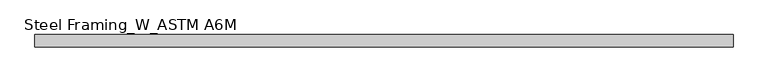
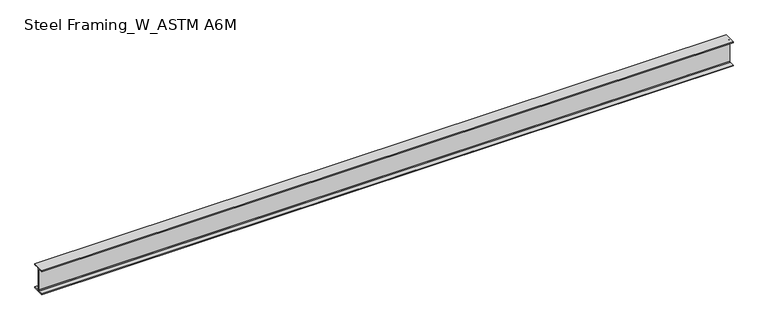
"""IFC4 building model written with IfcOpenShell, lengths in millimetres: beam geometry, Steel Framing_W_ASTM A6M : H_SB_AR_S02_W360x51_B4."""

from ifc_helpers import new_model, si_unit, point, frame, frame_2d, origin, place, context, project, spatial, polyline, circle_curve, trimmed, segment, composite_curve, outline, extrude, source, transform, mapped, element, save


def steel_framing_w_astm_a6m_e8746ce3(model_context):
    return source(origin(), model_context, "Body", "SweptSolid", [
        extrude(outline(composite_curve([segment(polyline([(85.5, -166.4), (85.5, -178.0), (-85.5, -178.0), (-85.5, -166.4), (-13.72, -166.4)]), True, "CONTINUOUS"), segment(trimmed(circle_curve(frame_2d((-13.72, -156.3)), 10.1), [point((-13.72, -166.4))], [point((-3.62, -156.3))], True, "CARTESIAN"), True, "CONTINUOUS"), segment(polyline([(-3.62, -156.3), (-3.62, 156.3)]), True, "CONTINUOUS"), segment(trimmed(circle_curve(frame_2d((-13.72, 156.3)), 10.1), [point((-3.62, 156.3))], [point((-13.72, 166.4))], True, "CARTESIAN"), True, "CONTINUOUS"), segment(polyline([(-13.72, 166.4), (-85.5, 166.4), (-85.5, 178.0), (85.5, 178.0), (85.5, 166.4), (13.72, 166.4)]), True, "CONTINUOUS"), segment(trimmed(circle_curve(frame_2d((13.72, 156.3)), 10.1), [point((13.72, 166.4))], [point((3.62, 156.3))], True, "CARTESIAN"), True, "CONTINUOUS"), segment(polyline([(3.62, 156.3), (3.62, -156.3)]), True, "CONTINUOUS"), segment(trimmed(circle_curve(frame_2d((13.72, -156.3)), 10.1), [point((3.62, -156.3))], [point((13.72, -166.4))], True, "CARTESIAN"), True, "CONTINUOUS"), segment(polyline([(13.72, -166.4), (85.5, -166.4)]), True, "CONTINUOUS")], self_intersect=False)), frame((-4901.8, 0.0, 0.0), z_axis=(1.0, 0.0, 0.0), x_axis=(0.0, 1.0, 0.0)), (0.0, 0.0, 1.0), 9715.9),
    ])


if __name__ == "__main__":
    model = new_model("IFC4")
    model_context = context("Model", 3, world=origin())
    ifc_project = project(units=[si_unit("LENGTHUNIT", "METRE", prefix="MILLI")], contexts=[model_context])
    site = spatial("IfcSite", under=ifc_project)
    building = spatial("IfcBuilding", under=site)
    placement = place(None, origin())
    steel_framing_w_astm_a6m_shape = steel_framing_w_astm_a6m_e8746ce3(model_context)
    element("IfcBeam", 1, ObjectType="Steel Framing_W_ASTM A6M : H_SB_AR_S02_W360x51_B4", at=placement, inside=building, context=model_context, shape_type="MappedRepresentation", body=[
        mapped(steel_framing_w_astm_a6m_shape, transform((0.0, 0.0, 0.0), x_axis=(1.0, 0.0, 0.0), y_axis=(0.0, 1.0, 0.0), z_axis=(0.0, 0.0, 1.0))),
    ])
    save(model, "model.ifc")

# Revit data of these elements
# Type "Steel Framing_W_ASTM A6M : H_SB_AR_S02_W360x51_B4"
#   Type Mark = "B4"
#   Section Name Key = "W14x34"
#   Width = 17.1 cm
#   Web Thickness = 0.724 cm
#   Web Fillet = 1.01 cm
#   Warping Constant = 287000.0 cm⁶
#   Torsional Moment of Inertia = 23.70 cm⁴
#   Section Area = 64.5 cm²
#   Plastic Modulus weak axis = 174.0 cm³
#   Plastic Modulus strong axis = 895.0 cm³
#   Perimeter = 1.36 m²/m
#   Nominal Weight = 51.00 kgf/m
#   Moment of Inertia weak axis = 970.00 cm⁴
#   Moment of Inertia strong axis = 14200.00 cm⁴
#   Height = 35.6 cm
#   Flange Thickness = 1.16 cm
#   Elastic Modulus weak axis = 113.0 cm³
#   Elastic Modulus strong axis = 796.0 cm³
#   Centroid Vertical = 17.8 cm
#   Centroid Horizontal = 8.55 cm
#   Length [instance default] = 1500 mm
#   Structural Material [instance default] = Steel, 45-345
#   Bolt Spacing = 0
#   Assembly Code = ""
# Element 1 (IfcBeam, "Steel Framing_W_ASTM A6M : H_SB_AR_S02_W360x51_B4")
#   Materials on its faces: "Steel, 45-345"
# Materials
#   "Steel, 45-345": class "Metal", colour RGB 189 187 185, transparency 0, Description = "Steel 345 MPa", Cost = 0
